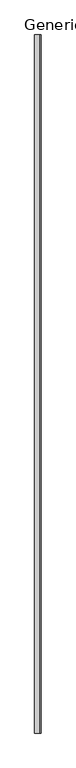
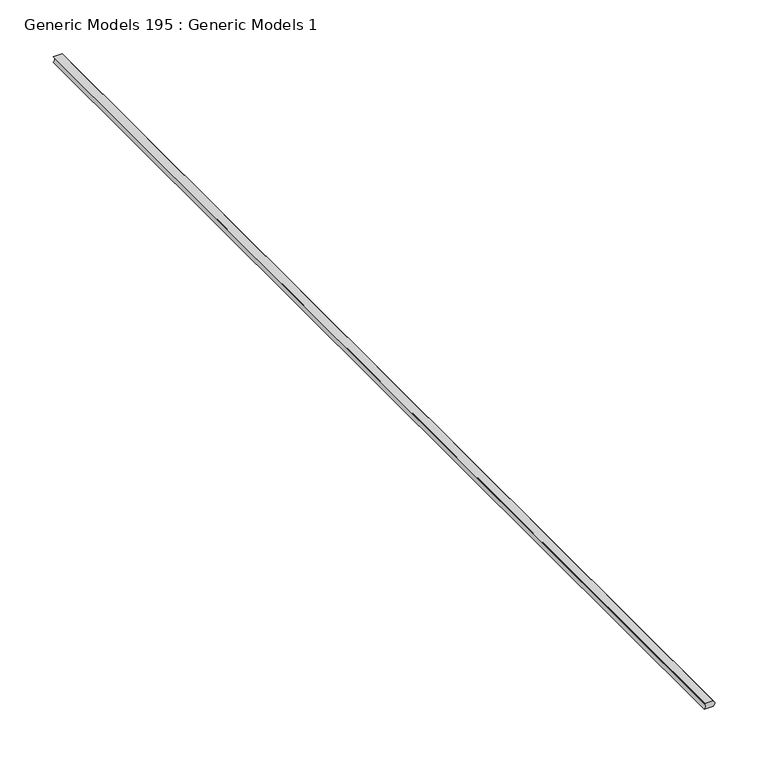
"""IFC4 building model written with IfcOpenShell, lengths in millimetres: proxy geometry, Generic Models 195 : Generic Models 1."""

from ifc_helpers import new_model, si_unit, point, frame, frame_2d, origin, place, context, project, spatial, polyline, circle_curve, trimmed, segment, composite_curve, outline, extrude, source, transform, mapped, element, save


def generic_models_195_generic_models_1_445a21b3(model_context):
    return source(origin(), model_context, "Body", "SweptSolid", [
        extrude(outline(composite_curve([segment(polyline([(-1924.4473206, 52542.4946108), (-1924.4473206, 52552.0196108)]), True, "CONTINUOUS"), segment(trimmed(circle_curve(frame_2d((-1921.2723206, 52549.1048703)), 4.3100275), [point((-1924.4473206, 52552.0196108))], [point((-1918.0973206, 52552.0196108))], False, "CARTESIAN"), True, "CONTINUOUS"), segment(polyline([(-1918.0973206, 52552.0196108), (-1918.0973206, 52542.4946108)]), True, "CONTINUOUS"), segment(trimmed(circle_curve(frame_2d((-1921.2723206, 52539.5798703)), 4.3100275), [point((-1918.0973206, 52542.4946108))], [point((-1924.4473206, 52542.4946108))], True, "CARTESIAN"), True, "CONTINUOUS")], self_intersect=False)), frame((0.0, 0.0, 0.0), z_axis=(0.0, 1.0, 0.0), x_axis=(0.0, 0.0, 1.0)), (0.0, 0.0, 1.0), 1219.2),
    ])


if __name__ == "__main__":
    model = new_model("IFC4")
    model_context = context("Model", 3, world=origin())
    ifc_project = project(units=[si_unit("LENGTHUNIT", "METRE", prefix="MILLI")], contexts=[model_context])
    site = spatial("IfcSite", under=ifc_project)
    building = spatial("IfcBuilding", under=site)
    placement = place(None, origin())
    generic_models_195_generic_models_1_shape = generic_models_195_generic_models_1_445a21b3(model_context)
    element("IfcBuildingElementProxy", 1, Name="Generic Models 195 : Generic Models 1", ObjectType="Generic Models 195 : Generic Models 1", at=placement, inside=building, context=model_context, shape_type="MappedRepresentation", body=[
        mapped(generic_models_195_generic_models_1_shape, transform((0.0, 0.0, 0.0), x_axis=(1.0, 0.0, 0.0), y_axis=(0.0, 1.0, 0.0), z_axis=(0.0, 0.0, 1.0))),
    ])
    save(model, "model.ifc")

# Revit data of these elements
# Element 1 (IfcBuildingElementProxy, "Generic Models 195 : Generic Models 1")
#   Materials on its faces: "ACOUSTICAL SEALANT"
# Materials
#   "ACOUSTICAL SEALANT": class "Unassigned", colour RGB 120 120 120, transparency 0, Cost = 0
